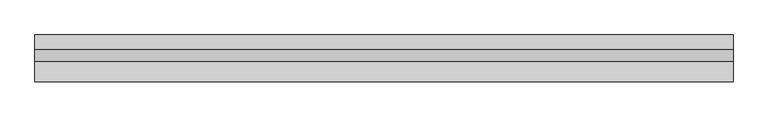
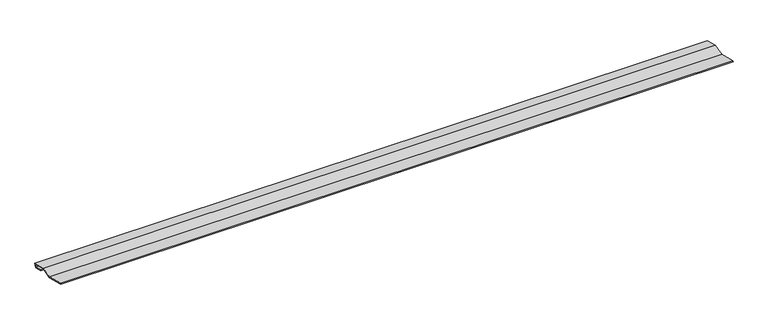
"""IFC4 building model written with IfcOpenShell, lengths in millimetres: proxy geometry, Gutter @ Roof003 : Gutter @ Roof003."""

from ifc_helpers import new_model, si_unit, frame, origin, place, context, project, spatial, polyline, outline, extrude, source, transform, mapped, element, save


def generic_models_fce577c4(model_context):
    return source(origin(), model_context, "Body", "SweptSolid", [
        extrude(outline(polyline([(4232.6081859, 41537.1432519), (4264.6308278, 41545.2330185), (4307.7733235, 41534.0387117), (4304.5942454, 41521.7866475), (4276.7109037, 41528.99344), (4277.346511, 41531.4526275), (4302.7729929, 41524.8808407), (4304.6868002, 41532.256592), (4264.623647, 41542.6114064), (4232.6010052, 41534.5216398), (4173.5378425, 41549.7872402), (4174.1734497, 41552.2464278), (4232.6081859, 41537.1432519)])), frame((255.0171875, 0.0, 0.0), z_axis=(1.0, 0.0, 0.0), x_axis=(0.0, 1.0, 0.0)), (0.0, 0.0, 1.0), 1999.85),
    ])


if __name__ == "__main__":
    model = new_model("IFC4")
    model_context = context("Model", 3, world=origin())
    ifc_project = project(units=[si_unit("LENGTHUNIT", "METRE", prefix="MILLI")], contexts=[model_context])
    site = spatial("IfcSite", under=ifc_project)
    building = spatial("IfcBuilding", under=site)
    placement = place(None, origin())
    generic_models_shape = generic_models_fce577c4(model_context)
    element("IfcBuildingElementProxy", 1, Name="Gutter @ Roof003 : Gutter @ Roof003", ObjectType="Gutter @ Roof003 : Gutter @ Roof003", at=placement, inside=building, context=model_context, shape_type="MappedRepresentation", body=[
        mapped(generic_models_shape, transform((0.0, 0.0, 0.0), x_axis=(1.0, 0.0, 0.0), y_axis=(0.0, 1.0, 0.0), z_axis=(0.0, 0.0, 1.0))),
    ])
    save(model, "model.ifc")

# Revit data of these elements
# Type "Gutter @ Roof003 : Gutter @ Roof003"
#   NameOverride = "Gutter @ Roof003"
# Element 1 (IfcBuildingElementProxy, "Gutter @ Roof003 : Gutter @ Roof003")
#   Materials on its faces: "CONT. SEAMLESS 16 GA COPPER BRAKE METAL GUTTER"
# Materials
#   "CONT. SEAMLESS 16 GA COPPER BRAKE METAL GUTTER": class "Unassigned", colour RGB 128 128 128, transparency 0
